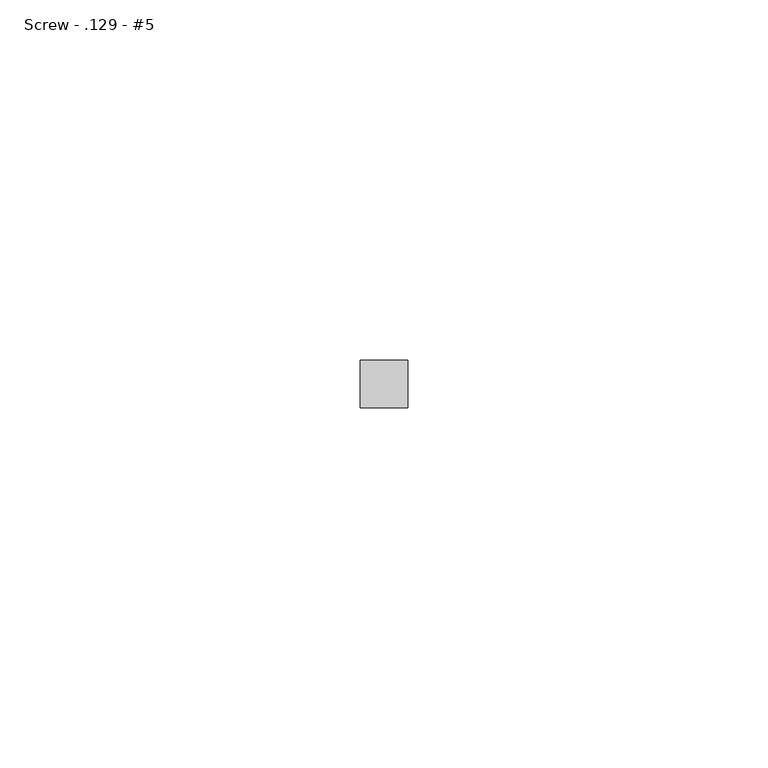
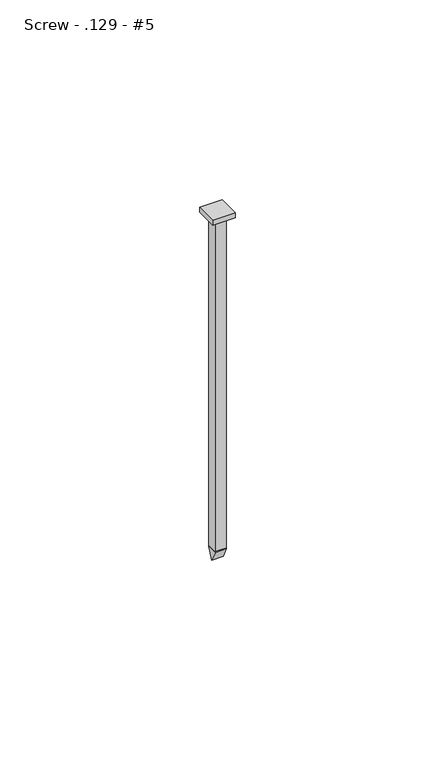
"""IFC4 building model written with IfcOpenShell, lengths in millimetres: fastener geometry, 060523 - W_P_C - Fastenings - Generic - SQUARE : Screw - .129 - #5."""

from ifc_helpers import new_model, si_unit, frame, origin, origin_with_axes, place, context, project, spatial, polyline, outline, extrude, source, transform, mapped, element, save


def screw_129_5_18eb6ddd(model_context):
    return source(origin(), model_context, "Body", "SweptSolid", [
        extrude(outline(polyline([(0.0, -104.8766), (-1.6383, -101.6), (1.6383, -101.6), (0.0, -104.8766)])), frame((-1.6383, 0.0, 0.0), z_axis=(1.0, 0.0, 0.0), x_axis=(0.0, 1.0, 0.0)), (0.0, 0.0, 1.0), 3.2766),
        extrude(outline(polyline([(-3.2766, -3.2766), (-3.2766, 3.2766), (3.2766, 3.2766), (3.2766, -3.2766), (-3.2766, -3.2766)])), origin_with_axes(), (0.0, 0.0, 1.0), 1.6383),
        extrude(outline(polyline([(-1.6383, 1.6383), (1.6383, 1.6383), (1.6383, -1.6383), (-1.6383, -1.6383), (-1.6383, 1.6383)])), frame((0.0, 0.0, -101.6), z_axis=(0.0, 0.0, 1.0), x_axis=(1.0, 0.0, 0.0)), (0.0, 0.0, 1.0), 101.6),
    ])


if __name__ == "__main__":
    model = new_model("IFC4")
    model_context = context("Model", 3, world=origin())
    ifc_project = project(units=[si_unit("LENGTHUNIT", "METRE", prefix="MILLI")], contexts=[model_context])
    site = spatial("IfcSite", under=ifc_project)
    building = spatial("IfcBuilding", under=site)
    placement = place(None, origin())
    screw_129_5_shape = screw_129_5_18eb6ddd(model_context)
    element("IfcFastener", 1, ObjectType="060523 - W_P_C - Fastenings - Generic - SQUARE : Screw - .129 - #5", at=placement, inside=building, context=model_context, shape_type="MappedRepresentation", body=[
        mapped(screw_129_5_shape, transform((0.0, 0.0, 0.0), x_axis=(1.0, 0.0, 0.0), y_axis=(0.0, 1.0, 0.0), z_axis=(0.0, 0.0, 1.0))),
    ])
    save(model, "model.ifc")

# Revit data of these elements
# Type "060523 - W_P_C - Fastenings - Generic - SQUARE : Screw - .129 - #5"
#   Washer_Thickness = 0' - 0.00333"
#   Washer Radius = 0' - 0.0745"
#   Washer Offset - Head = 0' - 0"
#   Washer Offset = 0' - 0"
#   Thickness_of_Substrate [instance default] = 0' - 1"
#   Side = 0' - 0 37/64"
#   Radius = 0' - 0.0645"
#   Length [instance default] = 0' - 4"
#   Head Size = 0' - 1"
#   Head Radius = 0' - 0 1/2"
#   Head Height = 0' - 0.01"
#   Double Diameter = 0' - 0.258"
#   Diameter = 0' - 0.129"
#   Default Elevation = 4' - 0"
#   Washer_Nut_Visibility = no
#   Washer_Head_Visibility = no
#   Round_Head_Visibility = yes
#   Point Visibility = yes
#   Nut_Visibility = no
#   Hex_Head_Visiblilty = no
#   Washer Material = none
#   Bolt Material (Size) = AT SILL - FASTENER AT 24" O.C.
# Materials
#   "AT SILL - FASTENER AT 24\" O.C.": class "Generic", colour RGB 120 120 120, transparency 0, Cost = 0
